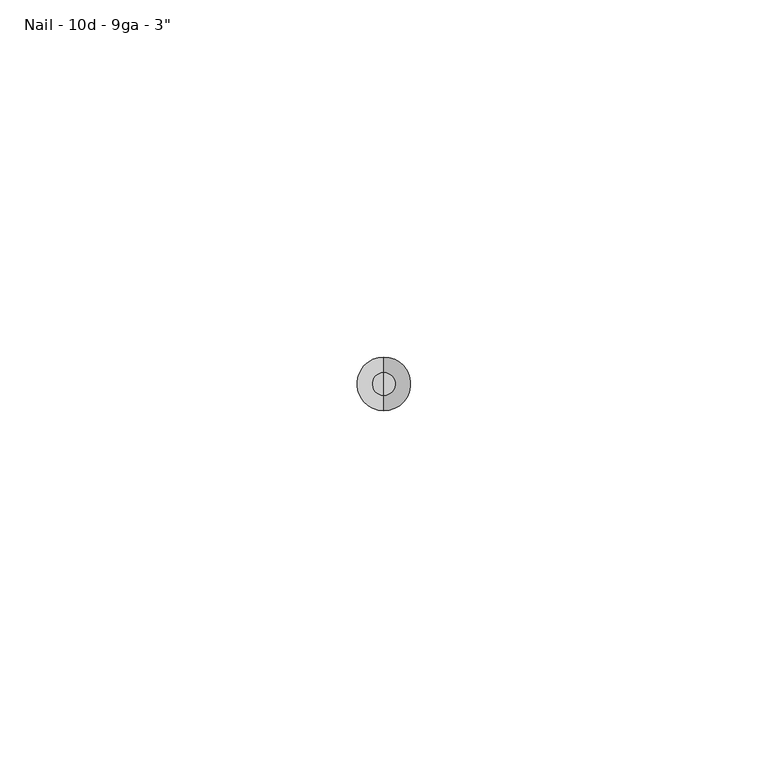
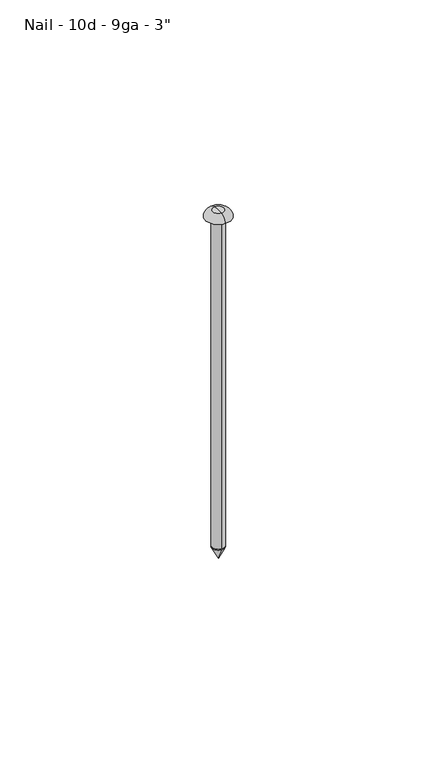
"""IFC4 building model written with IfcOpenShell, lengths in millimetres: fastener geometry."""

from ifc_helpers import new_model, si_unit, point, frame, origin, origin_2d, place, context, project, spatial, polyline, circle_curve, ellipse_curve, trimmed, segment, composite_curve, outline, extrude, source, transform, mapped, element, save
from ifc_brep_helpers import plane_surface, revolved_surface, advanced_brep


def fastener_3da11dce(model_context):
    return source(origin(), model_context, "Body", "SolidModel", [
        advanced_brep(
        [(0.0, -1.8796, -101.6), (0.0, 1.8796, -101.6), (0.0, 0.0, -101.6), (0.0, 0.0, -105.3592)],
        [
            (0, 1, circle_curve(frame((0.0, 0.0, -101.6), z_axis=(0.0, 0.0, 1.0), x_axis=(0.0, 1.0, 0.0)), 1.8796)),
            (1, 2),
            (2, 0),
            (1, 0, circle_curve(frame((0.0, 0.0, -101.6), z_axis=(0.0, 0.0, 1.0), x_axis=(0.0, 1.0, 0.0)), 1.8796)),
            (3, 1),
            (0, 3),
        ],
        [
            plane_surface(frame((0.0, 0.0, -101.6), z_axis=(0.0, 0.0, 1.0), x_axis=(0.0, 1.0, 0.0))),
            revolved_surface(polyline([(0.0, 1.8796, -101.6), (0.0, 0.0, -105.3592)]), (0.0, 0.0, -103.0840259), (0.0, 0.0, -1.0)),
        ],
        [
            (0, [[1, 2, 3]]),
            (0, [[4, -3, -2]]),
            (1, [[5, -1, 6]]),
            (1, [[-6, -4, -5]]),
        ],
    ),
        advanced_brep(
        [(0.0, 3.7592, 0.0), (0.0, -3.7592, 0.0), (0.0, 0.0, 0.0), (0.0, 0.0, 1.8796), (0.0, -1.5875, 1.8796), (0.0, 1.5875, 1.8796)],
        [
            (0, 1, circle_curve(frame((0.0, 0.0, 0.0), z_axis=(0.0, 0.0, -1.0), x_axis=(0.0, -1.0, 0.0)), 3.7592)),
            (1, 2),
            (2, 0),
            (1, 0, circle_curve(frame((0.0, 0.0, 0.0), z_axis=(0.0, 0.0, -1.0), x_axis=(0.0, -1.0, 0.0)), 3.7592)),
            (3, 4),
            (4, 5, circle_curve(frame((0.0, 0.0, 1.8796), z_axis=(0.0, 0.0, 1.0), x_axis=(0.0, -1.0, 0.0)), 1.5875)),
            (5, 3),
            (5, 4, circle_curve(frame((0.0, 0.0, 1.8796), z_axis=(0.0, 0.0, 1.0), x_axis=(0.0, -1.0, 0.0)), 1.5875)),
            (4, 1, circle_curve(frame((0.0, -1.5875, -0.314797), z_axis=(1.0, 0.0, 0.0), x_axis=(0.0, -1.0, 0.0)), 2.194397)),
            (0, 5, circle_curve(frame((0.0, 1.5875, -0.314797), z_axis=(1.0, 0.0, 0.0), x_axis=(0.0, 1.0, 0.0)), 2.194397)),
        ],
        [
            plane_surface(frame((0.0, 0.0, 0.0), z_axis=(0.0, 0.0, -1.0), x_axis=(0.0, -1.0, 0.0))),
            plane_surface(frame((0.0, 0.0, 1.8796), z_axis=(0.0, 0.0, 1.0), x_axis=(0.0, -1.0, 0.0))),
            revolved_surface(trimmed(ellipse_curve(frame((0.0, -1.5875, -0.314797), z_axis=(-1.0, 0.0, 0.0), x_axis=(0.0, -1.0, 0.0)), 2.194397, 2.194397), [point((0.0, -3.7592, 0.0))], [point((0.0, -1.5875, 1.8796))], True, "CARTESIAN"), (0.0, 0.0, 1.4840259), (0.0, 0.0, 1.0)),
        ],
        [
            (0, [[1, 2, 3]]),
            (0, [[4, -3, -2]]),
            (1, [[5, 6, 7]]),
            (1, [[-7, 8, -5]]),
            (2, [[-6, 9, -1, 10]]),
            (2, [[-8, -10, -4, -9]]),
        ],
    ),
        extrude(outline(composite_curve([segment(trimmed(circle_curve(origin_2d(), 1.8796), [point((0.0, -1.8796))], [point((0.0, 1.8796))], False, "CARTESIAN"), True, "CONTINUOUS"), segment(trimmed(circle_curve(origin_2d(), 1.8796), [point((0.0, 1.8796))], [point((0.0, -1.8796))], False, "CARTESIAN"), True, "CONTINUOUS")], self_intersect=False)), frame((0.0, 0.0, -101.6), z_axis=(0.0, 0.0, 1.0), x_axis=(1.0, 0.0, 0.0)), (0.0, 0.0, 1.0), 101.6),
    ])


if __name__ == "__main__":
    model = new_model("IFC4")
    model_context = context("Model", 3, world=origin())
    ifc_project = project(units=[si_unit("LENGTHUNIT", "METRE", prefix="MILLI")], contexts=[model_context])
    site = spatial("IfcSite", under=ifc_project)
    building = spatial("IfcBuilding", under=site)
    placement = place(None, origin())
    fastener_shape = fastener_3da11dce(model_context)
    element("IfcFastener", 1, ObjectType="060523 - W_P_C - Fastenings - Generic : Nail - 10d - 9ga - 3\"", at=placement, inside=building, context=model_context, shape_type="MappedRepresentation", body=[
        mapped(fastener_shape, transform((0.0, 0.0, 0.0), x_axis=(1.0, 0.0, 0.0), y_axis=(0.0, 1.0, 0.0), z_axis=(0.0, 0.0, 1.0))),
    ])
    save(model, "model.ifc")

# Revit data of these elements
# Type "060523 - W_P_C - Fastenings - Generic : Nail - 10d - 9ga - 3\""
#   Washer_Thickness = 0' - 0.00333"
#   Washer Radius = 0' - 0.084"
#   Washer Offset - Head = 0' - 0"
#   Washer Offset = 0' - 0"
#   Thickness_of_Substrate [instance default] = 0' - 1"
#   Side = 0' - 0 37/64"
#   Radius = 0' - 0.074"
#   Length [instance default] = 0' - 3"
#   Head Size = 0' - 1"
#   Head Radius = 0' - 0 1/2"
#   Head Height = 0' - 0.01"
#   Double Diameter = 0' - 0.296"
#   Diameter = 0' - 0.148"
#   Default Elevation = 4' - 0"
#   Washer_Nut_Visibility = no
#   Washer_Head_Visibility = no
#   Round_Head_Visibility = yes
#   Point Visibility = yes
#   Nut_Visibility = no
#   Hex_Head_Visiblilty = no
#   Washer Material = none
#   Bolt Material (Size) = AT SILL - FASTENER AT 24" O.C.
# Element 1 (IfcFastener, "060523 - W_P_C - Fastenings - Generic : Nail - 10d - 9ga - 3\"")
#   Length = 0' - 4"
#   Materials on its faces: "AT SILL - FASTENER AT 24\" O.C."
# Materials
#   "AT SILL - FASTENER AT 24\" O.C.": class "Generic", colour RGB 120 120 120, transparency 0, Cost = 0
